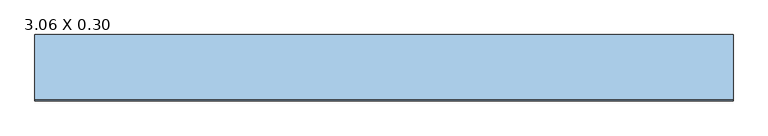
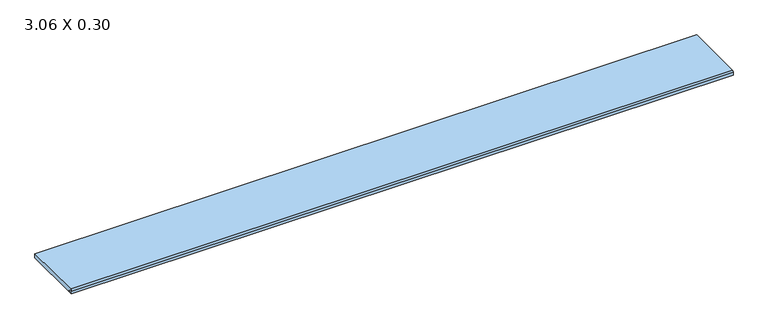
"""IFC4 building model written with IfcOpenShell, lengths in millimetres: window geometry, .CC_ND 300_PEDRA_PEITORIL RETO : 3.06 X 0.30."""

from ifc_helpers import new_model, si_unit, point, frame, frame_2d, origin, place, context, project, spatial, polyline, circle_curve, trimmed, segment, composite_curve, outline, extrude, source, transform, mapped, element, save


def window_3_06_x_0_30_1a8a3462(model_context):
    return source(origin(), model_context, "Body", "SweptSolid", [
        extrude(outline(composite_curve([segment(polyline([(-132.5083081, 1480.0), (-132.5083081, 1488.1993124), (-137.2619526, 1488.1993124), (-137.2619526, 1480.0), (-148.0, 1480.0), (-148.0, 1493.3808343)]), True, "CONTINUOUS"), segment(trimmed(circle_curve(frame_2d((-141.3808343, 1493.3808343)), 6.6191657), [point((-148.0, 1493.3808343))], [point((-141.3808343, 1500.0))], False, "CARTESIAN"), True, "CONTINUOUS"), segment(polyline([(-141.3808343, 1500.0), (143.7, 1500.0), (143.7, 1480.0), (-132.5083081, 1480.0)]), True, "CONTINUOUS")], self_intersect=False)), frame((-1530.0, 0.0, 0.0), z_axis=(1.0, 0.0, 0.0), x_axis=(0.0, 1.0, 0.0)), (0.0, 0.0, 1.0), 3060.0),
    ])


if __name__ == "__main__":
    model = new_model("IFC4")
    model_context = context("Model", 3, world=origin())
    ifc_project = project(units=[si_unit("LENGTHUNIT", "METRE", prefix="MILLI")], contexts=[model_context])
    site = spatial("IfcSite", under=ifc_project)
    building = spatial("IfcBuilding", under=site)
    placement = place(None, origin())
    window_3_06_x_0_30_shape = window_3_06_x_0_30_1a8a3462(model_context)
    element("IfcWindow", 1, ObjectType=".CC_ND 300_PEDRA_PEITORIL RETO : 3.06 X 0.30", at=placement, inside=building, context=model_context, shape_type="MappedRepresentation", body=[
        mapped(window_3_06_x_0_30_shape, transform((0.0, 0.0, 0.0), x_axis=(1.0, 0.0, 0.0), y_axis=(0.0, 1.0, 0.0), z_axis=(0.0, 0.0, 1.0))),
    ])
    save(model, "model.ifc")

# Revit data of these elements
# Type ".CC_ND 300_PEDRA_PEITORIL RETO : 3.06 X 0.30"
#   Type Mark = "70"
#   Largura da pedra [instance default] = 0.26 m
#   Extensão interior peitoril [instance default] = 0.03 m
#   Extensão exterior peitoril [instance default] = 0.03 m
#   Espessura = 0.02 m
#   Comprimento = 3.06 m
#   Altura-padrão do peitoril = 1.48 m
#   Peitoril = .GRANITO_BRANCO_ITAUNAS
#   Rough Width = 0
#   Rough Height = 0
#   Height = 0
#   Wall Closure = (empty or 0)
#   Width = 0
# Element 1 (IfcWindow, ".CC_ND 300_PEDRA_PEITORIL RETO : 3.06 X 0.30")
#   Largura da pedra = 0.2917 m
#   Extensão interior peitoril = 0.0257 m
#   Materials on its faces: ".GRANITO_BRANCO_ITAUNAS"
# Materials
#   ".GRANITO_BRANCO_ITAUNAS": class ".CC_PEDRA REVEST.", colour RGB 202 195 174, transparency 0, Description = "Revestimento em granito", Cost = 0
